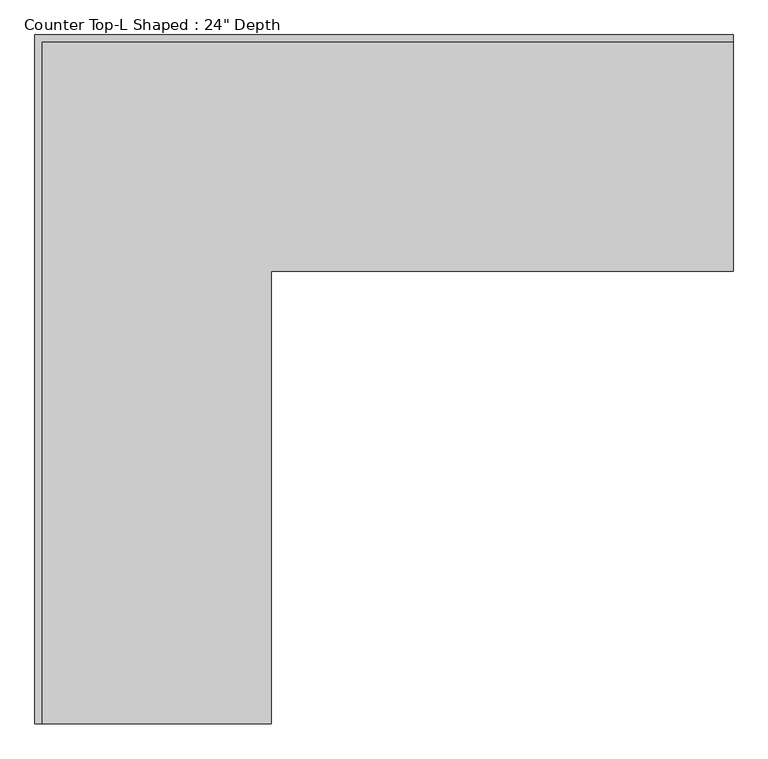
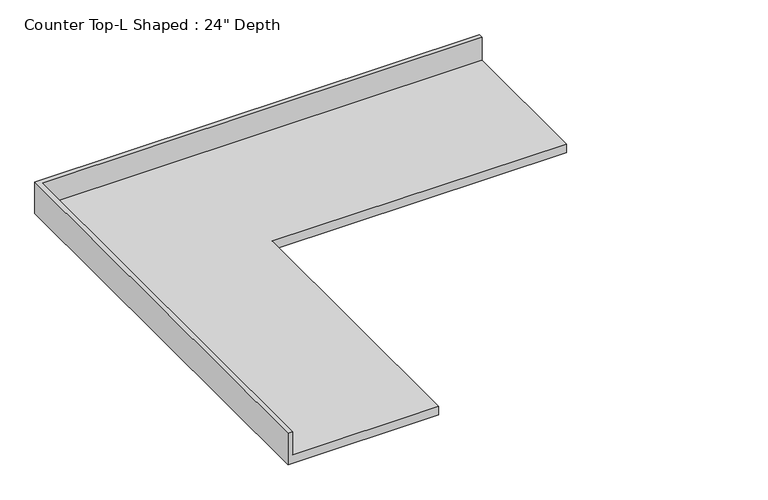
"""IFC4 building model written with IfcOpenShell, lengths in millimetres: furniture geometry."""

from ifc_helpers import new_model, si_unit, origin, place, context, project, spatial, faceted_brep, source, transform, mapped, element, save


def furniture_78cc8150(model_context):
    return source(origin(), model_context, "Body", "Brep", [
        faceted_brep([(-565.4622951, -1851.025, 914.4), (-565.4622951, -635.0, 914.4), (675.9627049, -635.0, 914.4), (675.9627049, -19.05, 914.4), (-1181.4122951, -19.05, 914.4), (-1181.4122951, -1851.025, 914.4), (675.9627049, 0.0, 876.3), (675.9627049, -635.0, 876.3), (-565.4622951, -635.0, 876.3), (-565.4622951, -1851.025, 876.3), (-1200.4622951, -1851.025, 876.3), (-1200.4622951, 0.0, 876.3), (-1200.4622951, 0.0, 1016.0), (675.9627049, 0.0, 1016.0), (-1200.4622951, -1851.025, 1016.0), (-1181.4122951, -1851.025, 1016.0), (675.9627049, -19.05, 1016.0), (-1181.4122951, -19.05, 1016.0)], [[[0, 1, 2, 3, 4, 5]], [[6, 7, 8, 9, 10, 11]], [[6, 11, 12, 13]], [[11, 10, 14, 12]], [[14, 10, 9, 0, 5, 15]], [[1, 0, 9, 8]], [[2, 1, 8, 7]], [[7, 6, 13, 16, 3, 2]], [[12, 14, 15, 17, 16, 13]], [[3, 16, 17, 4]], [[17, 15, 5, 4]]]),
    ])


if __name__ == "__main__":
    model = new_model("IFC4")
    model_context = context("Model", 3, world=origin())
    ifc_project = project(units=[si_unit("LENGTHUNIT", "METRE", prefix="MILLI")], contexts=[model_context])
    site = spatial("IfcSite", under=ifc_project)
    building = spatial("IfcBuilding", under=site)
    placement = place(None, origin())
    furniture_shape = furniture_78cc8150(model_context)
    element("IfcFurniture", 1, ObjectType="Counter Top-L Shaped : 24\" Depth", at=placement, inside=building, context=model_context, shape_type="MappedRepresentation", body=[
        mapped(furniture_shape, transform((0.0, 0.0, 0.0), x_axis=(1.0, 0.0, 0.0), y_axis=(0.0, 1.0, 0.0), z_axis=(0.0, 0.0, 1.0))),
    ])
    save(model, "model.ifc")

# Revit data of these elements
# Type "Counter Top-L Shaped : 24\" Depth"
#   Assembly Code = "C1030400"
#   Counter Thickness = 0' - 1 1/2"
#   Depth = 2' - 1"
#   Height = 3' - 0"
#   Length - Leg 1 [instance default] = 8' - 0"
#   Length - Leg 2 [instance default] = 6' - 0"
#   Counter Top Material = none
#   Default Elevation = 0
# Element 1 (IfcFurniture, "Counter Top-L Shaped : 24\" Depth")
#   Length - Leg 1 = 6' - 1 7/8"
#   Length - Leg 2 = 6' - 0 7/8"
#   Materials on its faces: "Counter Top"
# Materials
#   "Counter Top": class "Wood", colour RGB 226 177 128, transparency 0
